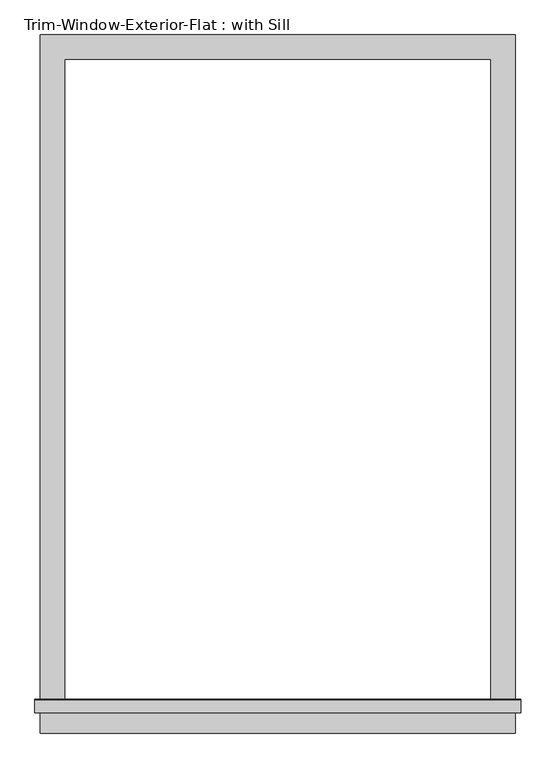
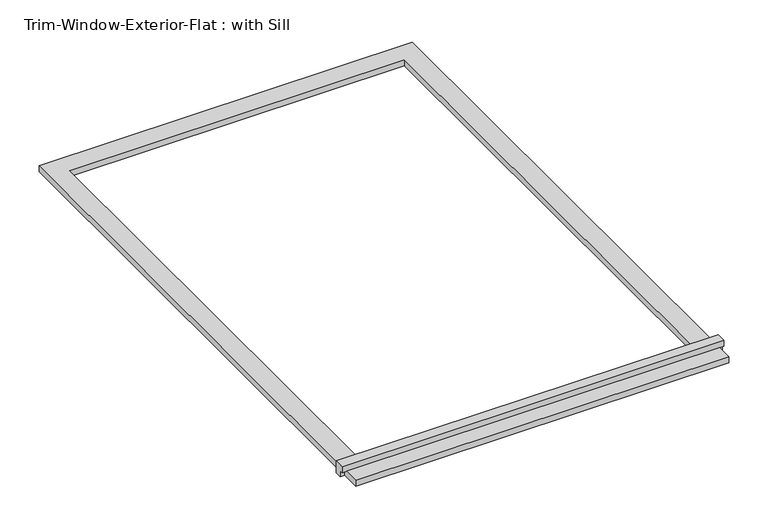
"""IFC4 building model written with IfcOpenShell, lengths in millimetres: proxy geometry, Trim-Window-Exterior-Flat : with Sill."""

from ifc_helpers import new_model, si_unit, frame, origin, origin_with_axes, place, context, project, spatial, polyline, outline, extrude, source, transform, mapped, element, save


def trim_window_exterior_flat_with_sill_5e7662e2(model_context):
    return source(origin(), model_context, "Body", "SweptSolid", [
        extrude(outline(polyline([(557.15, -1522.1823709), (557.15, -1579.3323709), (-557.15, -1579.3323709), (-557.15, -1522.1823709), (557.15, -1522.1823709)])), origin_with_axes(), (0.0, 0.0, 1.0), 19.05),
        extrude(outline(polyline([(-1531.75, 38.1), (-1502.4580645, 38.1), (-1500.0, 19.05), (-1500.0, 0.0), (-1522.1823709, 0.0), (-1522.1823709, 19.05), (-1531.75, 19.05), (-1531.75, 38.1)])), frame((-569.85, 0.0, 0.0), z_axis=(1.0, 0.0, 0.0), x_axis=(0.0, 1.0, 0.0)), (0.0, 0.0, 1.0), 1139.7),
        extrude(outline(polyline([(-557.15, 57.15), (557.15, 57.15), (557.15, -1500.0), (500.0, -1500.0), (500.0, 0.0), (-500.0, 0.0), (-500.0, -1500.0), (-557.15, -1500.0), (-557.15, 57.15)])), origin_with_axes(), (0.0, 0.0, 1.0), 19.05),
    ])


if __name__ == "__main__":
    model = new_model("IFC4")
    model_context = context("Model", 3, world=origin())
    ifc_project = project(units=[si_unit("LENGTHUNIT", "METRE", prefix="MILLI")], contexts=[model_context])
    site = spatial("IfcSite", under=ifc_project)
    building = spatial("IfcBuilding", under=site)
    placement = place(None, origin())
    trim_window_exterior_flat_with_sill_shape = trim_window_exterior_flat_with_sill_5e7662e2(model_context)
    element("IfcBuildingElementProxy", 1, Name="Trim-Window-Exterior-Flat : with Sill", ObjectType="Trim-Window-Exterior-Flat : with Sill", at=placement, inside=building, context=model_context, shape_type="MappedRepresentation", body=[
        mapped(trim_window_exterior_flat_with_sill_shape, transform((0.0, 0.0, 0.0), x_axis=(1.0, 0.0, 0.0), y_axis=(0.0, 1.0, 0.0), z_axis=(0.0, 0.0, 1.0))),
    ])
    save(model, "model.ifc")

# Revit data of these elements
# Type "Trim-Window-Exterior-Flat : with Sill"
#   Trim Width = 0.05715 m
#   Trim Thickness_Picture Frame = 0.03175 m
#   Trim Thickness_with Sill = 0.01905 m
#   Sill Thickness = 0.03175 m
#   Opening Width [instance default] = 0.6096 m
#   Opening Height [instance default] = 0.9144 m
#   Default Elevation = 1.2192 m
#   Sill = yes
#   Picture Frame = no
#   Trim Material [instance default] = none
# Element 1 (IfcBuildingElementProxy, "Trim-Window-Exterior-Flat : with Sill")
#   Opening Width = 1 m
#   Opening Height = 1.5 m
#   Trim Material = Clad - White
#   Materials on its faces: "Clad - White"
# Materials
#   "Clad - White": class "Wood", colour RGB 242 242 238, transparency 0, Cost = 0
